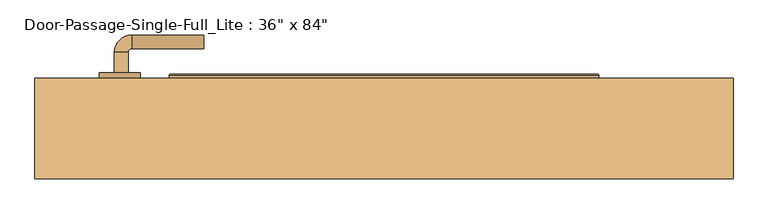
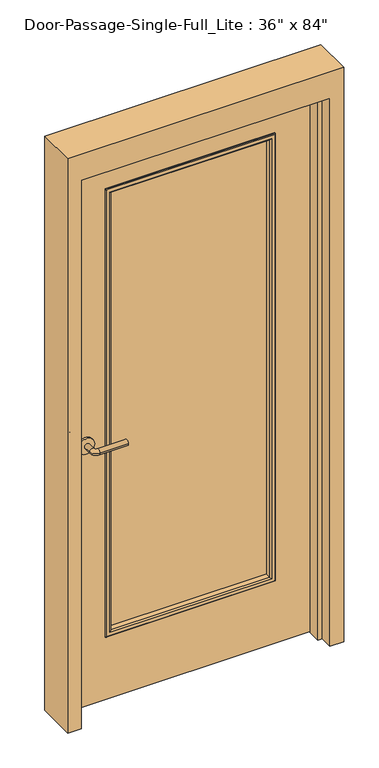
"""IFC4 building model written with IfcOpenShell, lengths in millimetres: door geometry."""

from ifc_helpers import new_model, si_unit, point, frame, frame_2d, origin, place, context, project, spatial, polyline, circle_curve, ellipse_curve, trimmed, segment, composite_curve, outline, extrude, faceted_brep, source, transform, mapped, element, save
from ifc_brep_helpers import plane_surface, cylinder_surface, revolved_surface, advanced_brep


def door_dac99271(model_context):
    return source(origin(), model_context, "Body", "SolidModel", [
        advanced_brep(
        [(-392.190625, 15.8125, 1016.0), (-372.190625, 15.8125, 1016.0), (-372.190625, -14.1875, 1016.0), (-392.190625, -14.1875, 1016.0), (-367.190625, -19.1875, 1016.0), (-367.190625, -39.1875, 1016.0), (-262.190625, -39.1875, 1016.0), (-262.190625, -19.1875, 1016.0)],
        [
            (0, 1, circle_curve(frame((-382.190625, 15.8125, 1016.0), z_axis=(0.0, 1.0, 0.0), x_axis=(1.0, 0.0, 0.0)), 10.0)),
            (1, 0, circle_curve(frame((-382.190625, 15.8125, 1016.0), z_axis=(0.0, 1.0, 0.0), x_axis=(1.0, 0.0, 0.0)), 10.0)),
            (1, 2),
            (2, 3, circle_curve(frame((-382.190625, -14.1875, 1016.0), z_axis=(0.0, 1.0, 0.0), x_axis=(1.0, 0.0, 0.0)), 10.0)),
            (3, 0),
            (3, 2, circle_curve(frame((-382.190625, -14.1875, 1016.0), z_axis=(0.0, 1.0, 0.0), x_axis=(1.0, 0.0, 0.0)), 10.0)),
            (4, 5, circle_curve(frame((-367.190625, -29.1875, 1016.0), z_axis=(-1.0, 0.0, 0.0), x_axis=(0.0, 1.0, 0.0)), 10.0)),
            (5, 3, circle_curve(frame((-367.190625, -14.1875, 1016.0), z_axis=(0.0, 0.0, -1.0), x_axis=(-1.0, 0.0, 0.0)), 25.0)),
            (2, 4, circle_curve(frame((-367.190625, -14.1875, 1016.0), z_axis=(0.0, 0.0, 1.0), x_axis=(-1.0, 0.0, 0.0)), 5.0)),
            (5, 4, circle_curve(frame((-367.190625, -29.1875, 1016.0), z_axis=(-1.0, 0.0, 0.0), x_axis=(0.0, 1.0, 0.0)), 10.0)),
            (6, 7, circle_curve(frame((-262.190625, -29.1875, 1016.0), z_axis=(1.0, 0.0, 0.0), x_axis=(0.0, 1.0, 0.0)), 10.0)),
            (7, 6, circle_curve(frame((-262.190625, -29.1875, 1016.0), z_axis=(1.0, 0.0, 0.0), x_axis=(0.0, 1.0, 0.0)), 10.0)),
            (4, 7),
            (6, 5),
        ],
        [
            plane_surface(frame((-382.190625, 15.8125, 1016.0), z_axis=(0.0, 1.0, 0.0), x_axis=(0.0, 0.0, 1.0))),
            cylinder_surface(frame((-382.190625, 15.8125, 1016.0), z_axis=(0.0, 1.0, 0.0), x_axis=(1.0, 0.0, 0.0)), 10.0),
            revolved_surface(trimmed(ellipse_curve(frame((-382.190625, -14.1875, 1016.0), z_axis=(0.0, -1.0, 0.0), x_axis=(1.0, 0.0, 0.0)), 10.0, 10.0), [point((-392.190625, -14.1875, 1016.0))], [point((-372.190625, -14.1875, 1016.0))], True, "CARTESIAN"), (-367.190625, -14.1875, 1016.0), (0.0, 0.0, -1.0)),
            revolved_surface(trimmed(ellipse_curve(frame((-382.190625, -14.1875, 1016.0), z_axis=(0.0, -1.0, 0.0), x_axis=(1.0, 0.0, 0.0)), 10.0, 10.0), [point((-372.190625, -14.1875, 1016.0))], [point((-392.190625, -14.1875, 1016.0))], True, "CARTESIAN"), (-367.190625, -14.1875, 1016.0), (0.0, 0.0, -1.0)),
            plane_surface(frame((-262.190625, -29.1875, 1016.0), z_axis=(1.0, 0.0, 0.0), x_axis=(0.0, 0.0, 1.0))),
            cylinder_surface(frame((-367.190625, -29.1875, 1016.0), z_axis=(-1.0, 0.0, 0.0), x_axis=(0.0, 1.0, 0.0)), 10.0),
        ],
        [
            (0, [[1, 2]]),
            (1, [[3, 4, 5, -2]]),
            (1, [[-5, 6, -3, -1]]),
            (2, [[7, 8, -4, 9]]),
            (3, [[10, -9, -6, -8]]),
            (4, [[11, 12]]),
            (5, [[13, -11, 14, -7]]),
            (5, [[-14, -12, -13, -10]]),
        ],
    ),
        extrude(outline(composite_curve([segment(trimmed(circle_curve(frame_2d((1016.0, -384.690625)), 30.0), [point((1016.0, -414.690625))], [point((1016.0, -354.690625))], False, "CARTESIAN"), True, "CONTINUOUS"), segment(trimmed(circle_curve(frame_2d((1016.0, -384.690625)), 30.0), [point((1016.0, -354.690625))], [point((1016.0, -414.690625))], False, "CARTESIAN"), True, "CONTINUOUS")], self_intersect=False)), frame((0.0, 15.8125, 0.0), z_axis=(0.0, 1.0, 0.0), x_axis=(0.0, 0.0, 1.0)), (0.0, 0.0, 1.0), 8.0),
        advanced_brep(
        [(-392.190625, 76.2625, 1016.0), (-372.190625, 76.2625, 1016.0), (-392.190625, 106.2625, 1016.0), (-372.190625, 106.2625, 1016.0), (-367.190625, 111.2625, 1016.0), (-367.190625, 131.2625, 1016.0), (-262.190625, 131.2625, 1016.0), (-262.190625, 111.2625, 1016.0)],
        [
            (0, 1, circle_curve(frame((-382.190625, 76.2625, 1016.0), z_axis=(0.0, -1.0, 0.0), x_axis=(1.0, 0.0, 0.0)), 10.0)),
            (1, 0, circle_curve(frame((-382.190625, 76.2625, 1016.0), z_axis=(0.0, -1.0, 0.0), x_axis=(1.0, 0.0, 0.0)), 10.0)),
            (0, 2),
            (2, 3, circle_curve(frame((-382.190625, 106.2625, 1016.0), z_axis=(0.0, -1.0, 0.0), x_axis=(1.0, 0.0, 0.0)), 10.0)),
            (3, 1),
            (3, 2, circle_curve(frame((-382.190625, 106.2625, 1016.0), z_axis=(0.0, -1.0, 0.0), x_axis=(1.0, 0.0, 0.0)), 10.0)),
            (4, 3, circle_curve(frame((-367.190625, 106.2625, 1016.0), z_axis=(0.0, 0.0, 1.0), x_axis=(-1.0, 0.0, 0.0)), 5.0)),
            (2, 5, circle_curve(frame((-367.190625, 106.2625, 1016.0), z_axis=(0.0, 0.0, -1.0), x_axis=(-1.0, 0.0, 0.0)), 25.0)),
            (5, 4, circle_curve(frame((-367.190625, 121.2625, 1016.0), z_axis=(-1.0, 0.0, 0.0), x_axis=(0.0, -1.0, 0.0)), 10.0)),
            (4, 5, circle_curve(frame((-367.190625, 121.2625, 1016.0), z_axis=(-1.0, 0.0, 0.0), x_axis=(0.0, -1.0, 0.0)), 10.0)),
            (6, 7, circle_curve(frame((-262.190625, 121.2625, 1016.0), z_axis=(1.0, 0.0, 0.0), x_axis=(0.0, -1.0, 0.0)), 10.0)),
            (7, 6, circle_curve(frame((-262.190625, 121.2625, 1016.0), z_axis=(1.0, 0.0, 0.0), x_axis=(0.0, -1.0, 0.0)), 10.0)),
            (5, 6),
            (7, 4),
        ],
        [
            plane_surface(frame((-382.190625, 76.2625, 1016.0), z_axis=(0.0, -1.0, 0.0), x_axis=(0.0, 0.0, 1.0))),
            cylinder_surface(frame((-382.190625, 76.2625, 1016.0), z_axis=(0.0, -1.0, 0.0), x_axis=(1.0, 0.0, 0.0)), 10.0),
            revolved_surface(trimmed(ellipse_curve(frame((-382.190625, 106.2625, 1016.0), z_axis=(0.0, -1.0, 0.0), x_axis=(1.0, 0.0, 0.0)), 10.0, 10.0), [point((-392.190625, 106.2625, 1016.0))], [point((-372.190625, 106.2625, 1016.0))], True, "CARTESIAN"), (-367.190625, 106.2625, 1016.0), (0.0, 0.0, -1.0)),
            revolved_surface(trimmed(ellipse_curve(frame((-382.190625, 106.2625, 1016.0), z_axis=(0.0, -1.0, 0.0), x_axis=(1.0, 0.0, 0.0)), 10.0, 10.0), [point((-372.190625, 106.2625, 1016.0))], [point((-392.190625, 106.2625, 1016.0))], True, "CARTESIAN"), (-367.190625, 106.2625, 1016.0), (0.0, 0.0, -1.0)),
            plane_surface(frame((-262.190625, 121.2625, 1016.0), z_axis=(1.0, 0.0, 0.0), x_axis=(0.0, 0.0, 1.0))),
            cylinder_surface(frame((-367.190625, 121.2625, 1016.0), z_axis=(-1.0, 0.0, 0.0), x_axis=(0.0, -1.0, 0.0)), 10.0),
        ],
        [
            (0, [[1, 2]]),
            (1, [[-1, 3, 4, 5]]),
            (1, [[-2, -5, 6, -3]]),
            (2, [[7, -4, 8, 9]]),
            (3, [[-8, -6, -7, 10]]),
            (4, [[11, 12]]),
            (5, [[-9, 13, -12, 14]]),
            (5, [[-10, -14, -11, -13]]),
        ],
    ),
        extrude(outline(composite_curve([segment(trimmed(circle_curve(frame_2d((1016.0, -384.690625)), 30.0), [point((1016.0, -414.690625))], [point((1016.0, -354.690625))], False, "CARTESIAN"), True, "CONTINUOUS"), segment(trimmed(circle_curve(frame_2d((1016.0, -384.690625)), 30.0), [point((1016.0, -354.690625))], [point((1016.0, -414.690625))], False, "CARTESIAN"), True, "CONTINUOUS")], self_intersect=False)), frame((0.0, 68.2625, 0.0), z_axis=(0.0, 1.0, 0.0), x_axis=(0.0, 0.0, 1.0)), (0.0, 0.0, 1.0), 8.0),
        extrude(outline(polyline([(304.8, 42.8625), (-304.8, 42.8625), (-304.8, 49.2125), (304.8, 49.2125), (304.8, 42.8625)])), frame((0.0, 0.0, 254.0), z_axis=(0.0, 0.0, 1.0), x_axis=(1.0, 0.0, 0.0)), (0.0, 0.0, 1.0), 1727.2),
        faceted_brep([(457.2, 19.05, 0.0), (457.2, 68.2625, 0.0), (508.0, 68.2625, 0.0), (508.0, -77.7875, 0.0), (457.2, -77.7875, 0.0), (457.2, -28.575, 0.0), (441.325, -28.575, 0.0), (441.325, 19.05, 0.0), (457.2, 19.05, 2133.6), (457.2, 68.2625, 2133.6), (-457.2, 68.2625, 2133.6), (-457.2, 68.2625, 0.0), (-508.0, 68.2625, 0.0), (-508.0, 68.2625, 2235.2), (508.0, 68.2625, 2235.2), (508.0, -77.7875, 2235.2), (-508.0, -77.7875, 2235.2), (-508.0, -77.7875, 0.0), (-457.2, -77.7875, 0.0), (-457.2, -77.7875, 2133.6), (457.2, -77.7875, 2133.6), (457.2, -28.575, 2133.6), (-457.2, -28.575, 2133.6), (-457.2, -28.575, 0.0), (-441.325, -28.575, 0.0), (-441.325, -28.575, 2117.725), (441.325, -28.575, 2117.725), (441.325, 19.05, 2117.725), (-441.325, 19.05, 2117.725), (-441.325, 19.05, 0.0), (-457.2, 19.05, 0.0), (-457.2, 19.05, 2133.6)], [[[0, 1, 2, 3, 4, 5, 6, 7]], [[1, 0, 8, 9]], [[2, 1, 9, 10, 11, 12, 13, 14]], [[3, 2, 14, 15]], [[4, 3, 15, 16, 17, 18, 19, 20]], [[5, 4, 20, 21]], [[6, 5, 21, 22, 23, 24, 25, 26]], [[7, 6, 26, 27]], [[0, 7, 27, 28, 29, 30, 31, 8]], [[9, 8, 31, 10]], [[20, 19, 22, 21]], [[26, 25, 28, 27]], [[12, 11, 30, 29, 24, 23, 18, 17]], [[11, 10, 31, 30]], [[13, 12, 17, 16]], [[19, 18, 23, 22]], [[25, 24, 29, 28]], [[15, 14, 13, 16]]]),
        extrude(outline(polyline([(2133.6, -457.2), (0.0, -457.2), (0.0, 457.2), (2133.6, 457.2), (2133.6, -457.2)]), holes=[polyline([(1981.2, -304.8), (1981.2, 304.8), (254.0, 304.8), (254.0, -304.8), (1981.2, -304.8)])]), frame((0.0, 23.8125, 0.0), z_axis=(0.0, 1.0, 0.0), x_axis=(0.0, 0.0, 1.0)), (0.0, 0.0, 1.0), 44.45),
        advanced_brep(
        [(-304.8, 49.2125, 1981.2), (-304.8, 68.2625, 1981.2), (-304.8, 68.2625, 254.0), (-304.8, 49.2125, 254.0), (-292.8, 69.2625, 1969.2), (-292.8, 49.2125, 1969.2), (-292.8, 49.2125, 266.0), (-292.8, 69.2625, 266.0), (-297.8, 74.2625, 1974.2), (-297.8, 74.2625, 261.0), (-312.8, 72.2625, 1989.2), (-310.8, 74.2625, 1987.2), (-310.8, 74.2625, 248.0), (-312.8, 72.2625, 246.0), (-312.8, 68.2625, 1989.2), (-312.8, 68.2625, 246.0), (304.8, 68.2625, 254.0), (304.8, 49.2125, 254.0), (292.8, 49.2125, 266.0), (292.8, 69.2625, 266.0), (297.8, 74.2625, 261.0), (310.8, 74.2625, 248.0), (312.8, 72.2625, 246.0), (312.8, 68.2625, 246.0), (304.8, 68.2625, 1981.2), (304.8, 49.2125, 1981.2), (292.8, 49.2125, 1969.2), (292.8, 69.2625, 1969.2), (297.8, 74.2625, 1974.2), (310.8, 74.2625, 1987.2), (312.8, 72.2625, 1989.2), (312.8, 68.2625, 1989.2)],
        [
            (0, 1),
            (1, 2),
            (2, 3),
            (3, 0),
            (4, 5),
            (5, 6),
            (6, 7),
            (7, 4),
            (8, 4, ellipse_curve(frame((-297.8, 69.2625, 1974.2), z_axis=(-0.7071067811865475, 0.0, -0.7071067811865475), x_axis=(-0.7071067811865474, 0.0, 0.7071067811865476)), 7.0710678, 5.0)),
            (7, 9, ellipse_curve(frame((-297.8, 69.2625, 261.0), z_axis=(-0.7071067811865475, 0.0, 0.7071067811865475), x_axis=(0.7071067811865474, 0.0, 0.7071067811865476)), 7.0710678, 5.0)),
            (9, 8),
            (10, 11, ellipse_curve(frame((-310.8, 72.2625, 1987.2), z_axis=(-0.7071067811865475, 0.0, -0.7071067811865475), x_axis=(-0.7071067811865474, 0.0, 0.7071067811865476)), 2.8284271, 2.0)),
            (11, 12),
            (12, 13, ellipse_curve(frame((-310.8, 72.2625, 248.0), z_axis=(-0.7071067811865475, 0.0, 0.7071067811865475), x_axis=(0.7071067811865474, 0.0, 0.7071067811865476)), 2.8284271, 2.0)),
            (13, 10),
            (14, 10),
            (13, 15),
            (15, 14),
            (2, 16),
            (16, 17),
            (17, 3),
            (6, 18),
            (18, 19),
            (19, 7),
            (19, 20, ellipse_curve(frame((297.8, 69.2625, 261.0), z_axis=(-0.7071067811865475, 0.0, -0.7071067811865475), x_axis=(-0.7071067811865476, 0.0, 0.7071067811865474)), 7.0710678, 5.0)),
            (20, 9),
            (12, 21),
            (21, 22, ellipse_curve(frame((310.8, 72.2625, 248.0), z_axis=(-0.7071067811865475, 0.0, -0.7071067811865475), x_axis=(-0.7071067811865476, 0.0, 0.7071067811865474)), 2.8284271, 2.0)),
            (22, 13),
            (22, 23),
            (23, 15),
            (16, 24),
            (24, 25),
            (25, 17),
            (18, 26),
            (26, 27),
            (27, 19),
            (27, 28, ellipse_curve(frame((297.8, 69.2625, 1974.2), z_axis=(0.7071067811865475, 0.0, -0.7071067811865475), x_axis=(-0.7071067811865474, 0.0, -0.7071067811865476)), 7.0710678, 5.0)),
            (28, 20),
            (21, 29),
            (29, 30, ellipse_curve(frame((310.8, 72.2625, 1987.2), z_axis=(0.7071067811865475, 0.0, -0.7071067811865475), x_axis=(-0.7071067811865474, 0.0, -0.7071067811865476)), 2.8284271, 2.0)),
            (30, 22),
            (30, 31),
            (31, 23),
            (31, 14),
            (1, 24),
            (0, 25),
            (5, 26),
            (4, 27),
            (8, 28),
            (11, 29),
            (10, 30),
        ],
        [
            plane_surface(frame((-304.8, 68.2625, 1981.2), z_axis=(-1.0, 0.0, 0.0), x_axis=(0.0, 0.0, -1.0))),
            plane_surface(frame((-292.8, 49.2125, 1969.2), z_axis=(1.0, 0.0, 0.0), x_axis=(0.0, 0.0, -1.0))),
            cylinder_surface(frame((-297.8, 69.2625, 1981.2), z_axis=(0.0, 0.0, 1.0), x_axis=(-1.0, 0.0, 0.0)), 5.0),
            cylinder_surface(frame((-310.8, 72.2625, 1981.2), z_axis=(0.0, 0.0, 1.0), x_axis=(-1.0, 0.0, 0.0)), 2.0),
            plane_surface(frame((-312.8, 72.2625, 1989.2), z_axis=(-1.0, 0.0, 0.0), x_axis=(0.0, 0.0, -1.0))),
            plane_surface(frame((-304.8, 68.2625, 254.0), z_axis=(0.0, 0.0, -1.0), x_axis=(1.0, 0.0, 0.0))),
            plane_surface(frame((-292.8, 49.2125, 266.0), z_axis=(0.0, 0.0, 1.0), x_axis=(1.0, 0.0, 0.0))),
            cylinder_surface(frame((-304.8, 69.2625, 261.0), z_axis=(-1.0, 0.0, 0.0), x_axis=(0.0, 0.0, -1.0)), 5.0),
            cylinder_surface(frame((-304.8, 72.2625, 248.0), z_axis=(-1.0, 0.0, 0.0), x_axis=(0.0, 0.0, -1.0)), 2.0),
            plane_surface(frame((-312.8, 72.2625, 246.0), z_axis=(0.0, 0.0, -1.0), x_axis=(1.0, 0.0, 0.0))),
            plane_surface(frame((304.8, 68.2625, 254.0), z_axis=(1.0, 0.0, 0.0), x_axis=(0.0, 0.0, 1.0))),
            plane_surface(frame((292.8, 49.2125, 266.0), z_axis=(-1.0, 0.0, 0.0), x_axis=(0.0, 0.0, 1.0))),
            cylinder_surface(frame((297.8, 69.2625, 254.0), z_axis=(0.0, 0.0, -1.0), x_axis=(1.0, 0.0, 0.0)), 5.0),
            cylinder_surface(frame((310.8, 72.2625, 254.0), z_axis=(0.0, 0.0, -1.0), x_axis=(1.0, 0.0, 0.0)), 2.0),
            plane_surface(frame((312.8, 72.2625, 246.0), z_axis=(1.0, 0.0, 0.0), x_axis=(0.0, 0.0, 1.0))),
            plane_surface(frame((312.8, 68.2625, 1989.2), z_axis=(0.0, -1.0, 0.0), x_axis=(-1.0, 0.0, 0.0))),
            plane_surface(frame((304.8, 68.2625, 1981.2), z_axis=(0.0, 0.0, 1.0), x_axis=(-1.0, 0.0, 0.0))),
            plane_surface(frame((304.8, 49.2125, 1981.2), z_axis=(0.0, -1.0, 0.0), x_axis=(-1.0, 0.0, 0.0))),
            plane_surface(frame((292.8, 49.2125, 1969.2), z_axis=(0.0, 0.0, -1.0), x_axis=(-1.0, 0.0, 0.0))),
            cylinder_surface(frame((304.8, 69.2625, 1974.2), z_axis=(1.0, 0.0, 0.0), x_axis=(0.0, 0.0, 1.0)), 5.0),
            plane_surface(frame((297.8, 74.2625, 1974.2), z_axis=(0.0, 1.0, 0.0), x_axis=(-1.0, 0.0, 0.0))),
            cylinder_surface(frame((304.8, 72.2625, 1987.2), z_axis=(1.0, 0.0, 0.0), x_axis=(0.0, 0.0, 1.0)), 2.0),
            plane_surface(frame((312.8, 72.2625, 1989.2), z_axis=(0.0, 0.0, 1.0), x_axis=(-1.0, 0.0, 0.0))),
        ],
        [
            (0, [[1, 2, 3, 4]]),
            (1, [[5, 6, 7, 8]]),
            (2, [[9, -8, 10, 11]]),
            (3, [[12, 13, 14, 15]]),
            (4, [[16, -15, 17, 18]]),
            (5, [[-3, 19, 20, 21]]),
            (6, [[-7, 22, 23, 24]]),
            (7, [[-10, -24, 25, 26]]),
            (8, [[-14, 27, 28, 29]]),
            (9, [[-17, -29, 30, 31]]),
            (10, [[-20, 32, 33, 34]]),
            (11, [[-23, 35, 36, 37]]),
            (12, [[-25, -37, 38, 39]]),
            (13, [[-28, 40, 41, 42]]),
            (14, [[-30, -42, 43, 44]]),
            (15, [[-31, -44, 45, -18], [46, -32, -19, -2]]),
            (16, [[-33, -46, -1, 47]]),
            (17, [[-21, -34, -47, -4], [48, -35, -22, -6]]),
            (18, [[-36, -48, -5, 49]]),
            (19, [[-38, -49, -9, 50]]),
            (20, [[51, -40, -27, -13], [-26, -39, -50, -11]]),
            (21, [[-41, -51, -12, 52]]),
            (22, [[-43, -52, -16, -45]]),
        ],
    ),
        advanced_brep(
        [(-304.8, 42.8625, 254.0), (-304.8, 23.8125, 254.0), (-304.8, 23.8125, 1981.2), (-304.8, 42.8625, 1981.2), (-292.8, 22.8125, 266.0), (-292.8, 42.8625, 266.0), (-292.8, 42.8625, 1969.2), (-292.8, 22.8125, 1969.2), (-297.8, 17.8125, 261.0), (-297.8, 17.8125, 1974.2), (-312.8, 19.8125, 246.0), (-310.8, 17.8125, 248.0), (-310.8, 17.8125, 1987.2), (-312.8, 19.8125, 1989.2), (-312.8, 23.8125, 246.0), (-312.8, 23.8125, 1989.2), (304.8, 23.8125, 1981.2), (304.8, 42.8625, 1981.2), (292.8, 42.8625, 1969.2), (292.8, 22.8125, 1969.2), (297.8, 17.8125, 1974.2), (310.8, 17.8125, 1987.2), (312.8, 19.8125, 1989.2), (312.8, 23.8125, 1989.2), (304.8, 23.8125, 254.0), (304.8, 42.8625, 254.0), (292.8, 42.8625, 266.0), (292.8, 22.8125, 266.0), (297.8, 17.8125, 261.0), (310.8, 17.8125, 248.0), (312.8, 19.8125, 246.0), (312.8, 23.8125, 246.0)],
        [
            (0, 1),
            (1, 2),
            (2, 3),
            (3, 0),
            (4, 5),
            (5, 6),
            (6, 7),
            (7, 4),
            (8, 4, ellipse_curve(frame((-297.8, 22.8125, 261.0), z_axis=(-0.7071067811865475, 0.0, 0.7071067811865475), x_axis=(-0.7071067811865474, 0.0, -0.7071067811865476)), 7.0710678, 5.0)),
            (7, 9, ellipse_curve(frame((-297.8, 22.8125, 1974.2), z_axis=(-0.7071067811865475, 0.0, -0.7071067811865475), x_axis=(0.7071067811865474, 0.0, -0.7071067811865476)), 7.0710678, 5.0)),
            (9, 8),
            (10, 11, ellipse_curve(frame((-310.8, 19.8125, 248.0), z_axis=(-0.7071067811865475, 0.0, 0.7071067811865475), x_axis=(-0.7071067811865474, 0.0, -0.7071067811865476)), 2.8284271, 2.0)),
            (11, 12),
            (12, 13, ellipse_curve(frame((-310.8, 19.8125, 1987.2), z_axis=(-0.7071067811865475, 0.0, -0.7071067811865475), x_axis=(0.7071067811865474, 0.0, -0.7071067811865476)), 2.8284271, 2.0)),
            (13, 10),
            (14, 10),
            (13, 15),
            (15, 14),
            (2, 16),
            (16, 17),
            (17, 3),
            (6, 18),
            (18, 19),
            (19, 7),
            (19, 20, ellipse_curve(frame((297.8, 22.8125, 1974.2), z_axis=(-0.7071067811865475, 0.0, 0.7071067811865475), x_axis=(-0.7071067811865476, 0.0, -0.7071067811865474)), 7.0710678, 5.0)),
            (20, 9),
            (12, 21),
            (21, 22, ellipse_curve(frame((310.8, 19.8125, 1987.2), z_axis=(-0.7071067811865475, 0.0, 0.7071067811865475), x_axis=(-0.7071067811865476, 0.0, -0.7071067811865474)), 2.8284271, 2.0)),
            (22, 13),
            (22, 23),
            (23, 15),
            (16, 24),
            (24, 25),
            (25, 17),
            (18, 26),
            (26, 27),
            (27, 19),
            (27, 28, ellipse_curve(frame((297.8, 22.8125, 261.0), z_axis=(0.7071067811865475, 0.0, 0.7071067811865475), x_axis=(-0.7071067811865474, 0.0, 0.7071067811865476)), 7.0710678, 5.0)),
            (28, 20),
            (21, 29),
            (29, 30, ellipse_curve(frame((310.8, 19.8125, 248.0), z_axis=(0.7071067811865475, 0.0, 0.7071067811865475), x_axis=(-0.7071067811865474, 0.0, 0.7071067811865476)), 2.8284271, 2.0)),
            (30, 22),
            (30, 31),
            (31, 23),
            (31, 14),
            (1, 24),
            (0, 25),
            (5, 26),
            (4, 27),
            (8, 28),
            (11, 29),
            (10, 30),
        ],
        [
            plane_surface(frame((-304.8, 23.8125, 254.0), z_axis=(-1.0, 0.0, 0.0), x_axis=(0.0, 0.0, 1.0))),
            plane_surface(frame((-292.8, 42.8625, 266.0), z_axis=(1.0, 0.0, 0.0), x_axis=(0.0, 0.0, 1.0))),
            cylinder_surface(frame((-297.8, 22.8125, 254.0), z_axis=(0.0, 0.0, -1.0), x_axis=(-1.0, 0.0, 0.0)), 5.0),
            cylinder_surface(frame((-310.8, 19.8125, 254.0), z_axis=(0.0, 0.0, -1.0), x_axis=(-1.0, 0.0, 0.0)), 2.0),
            plane_surface(frame((-312.8, 19.8125, 246.0), z_axis=(-1.0, 0.0, 0.0), x_axis=(0.0, 0.0, 1.0))),
            plane_surface(frame((-304.8, 23.8125, 1981.2), z_axis=(0.0, 0.0, 1.0), x_axis=(1.0, 0.0, 0.0))),
            plane_surface(frame((-292.8, 42.8625, 1969.2), z_axis=(0.0, 0.0, -1.0), x_axis=(1.0, 0.0, 0.0))),
            cylinder_surface(frame((-304.8, 22.8125, 1974.2), z_axis=(-1.0, 0.0, 0.0), x_axis=(0.0, 0.0, 1.0)), 5.0),
            cylinder_surface(frame((-304.8, 19.8125, 1987.2), z_axis=(-1.0, 0.0, 0.0), x_axis=(0.0, 0.0, 1.0)), 2.0),
            plane_surface(frame((-312.8, 19.8125, 1989.2), z_axis=(0.0, 0.0, 1.0), x_axis=(1.0, 0.0, 0.0))),
            plane_surface(frame((304.8, 23.8125, 1981.2), z_axis=(1.0, 0.0, 0.0), x_axis=(0.0, 0.0, -1.0))),
            plane_surface(frame((292.8, 42.8625, 1969.2), z_axis=(-1.0, 0.0, 0.0), x_axis=(0.0, 0.0, -1.0))),
            cylinder_surface(frame((297.8, 22.8125, 1981.2), z_axis=(0.0, 0.0, 1.0), x_axis=(1.0, 0.0, 0.0)), 5.0),
            cylinder_surface(frame((310.8, 19.8125, 1981.2), z_axis=(0.0, 0.0, 1.0), x_axis=(1.0, 0.0, 0.0)), 2.0),
            plane_surface(frame((312.8, 19.8125, 1989.2), z_axis=(1.0, 0.0, 0.0), x_axis=(0.0, 0.0, -1.0))),
            plane_surface(frame((312.8, 23.8125, 246.0), z_axis=(0.0, 1.0, 0.0), x_axis=(-1.0, 0.0, 0.0))),
            plane_surface(frame((304.8, 23.8125, 254.0), z_axis=(0.0, 0.0, -1.0), x_axis=(-1.0, 0.0, 0.0))),
            plane_surface(frame((304.8, 42.8625, 254.0), z_axis=(0.0, 1.0, 0.0), x_axis=(-1.0, 0.0, 0.0))),
            plane_surface(frame((292.8, 42.8625, 266.0), z_axis=(0.0, 0.0, 1.0), x_axis=(-1.0, 0.0, 0.0))),
            cylinder_surface(frame((304.8, 22.8125, 261.0), z_axis=(1.0, 0.0, 0.0), x_axis=(0.0, 0.0, -1.0)), 5.0),
            plane_surface(frame((297.8, 17.8125, 261.0), z_axis=(0.0, -1.0, 0.0), x_axis=(-1.0, 0.0, 0.0))),
            cylinder_surface(frame((304.8, 19.8125, 248.0), z_axis=(1.0, 0.0, 0.0), x_axis=(0.0, 0.0, -1.0)), 2.0),
            plane_surface(frame((312.8, 19.8125, 246.0), z_axis=(0.0, 0.0, -1.0), x_axis=(-1.0, 0.0, 0.0))),
        ],
        [
            (0, [[1, 2, 3, 4]]),
            (1, [[5, 6, 7, 8]]),
            (2, [[9, -8, 10, 11]]),
            (3, [[12, 13, 14, 15]]),
            (4, [[16, -15, 17, 18]]),
            (5, [[-3, 19, 20, 21]]),
            (6, [[-7, 22, 23, 24]]),
            (7, [[-10, -24, 25, 26]]),
            (8, [[-14, 27, 28, 29]]),
            (9, [[-17, -29, 30, 31]]),
            (10, [[-20, 32, 33, 34]]),
            (11, [[-23, 35, 36, 37]]),
            (12, [[-25, -37, 38, 39]]),
            (13, [[-28, 40, 41, 42]]),
            (14, [[-30, -42, 43, 44]]),
            (15, [[-31, -44, 45, -18], [46, -32, -19, -2]]),
            (16, [[-33, -46, -1, 47]]),
            (17, [[-21, -34, -47, -4], [48, -35, -22, -6]]),
            (18, [[-36, -48, -5, 49]]),
            (19, [[-38, -49, -9, 50]]),
            (20, [[51, -40, -27, -13], [-26, -39, -50, -11]]),
            (21, [[-41, -51, -12, 52]]),
            (22, [[-43, -52, -16, -45]]),
        ],
    ),
    ])


if __name__ == "__main__":
    model = new_model("IFC4")
    model_context = context("Model", 3, world=origin())
    ifc_project = project(units=[si_unit("LENGTHUNIT", "METRE", prefix="MILLI")], contexts=[model_context])
    site = spatial("IfcSite", under=ifc_project)
    building = spatial("IfcBuilding", under=site)
    placement = place(None, origin())
    door_shape = door_dac99271(model_context)
    element("IfcDoor", 1, ObjectType="Door-Passage-Single-Full_Lite : 36\" x 84\"", at=placement, inside=building, context=model_context, shape_type="MappedRepresentation", body=[
        mapped(door_shape, transform((0.0, 0.0, 0.0), x_axis=(1.0, 0.0, 0.0), y_axis=(0.0, 1.0, 0.0), z_axis=(0.0, 0.0, 1.0))),
    ])
    save(model, "model.ifc")

# Revit data of these elements
# Type "Door-Passage-Single-Full_Lite : 36\" x 84\""
#   Type Mark = "52"
#   Assembly Code = "B2030100"
#   Analytic Construction = "Wooden"
#   Thickness = 0' - 1 3/4"
#   Thermal Resistance (R) = 2.5876 (h·ft²·°F)/BTU
#   Swing Angle [instance default] = 90.00°
#   Strike Height = 3' - 4"
#   Rough Width [instance default] = 3' - 4"
#   Rough Height [instance default] = 7' - 4"
#   MF Opening Height [instance default] = 0' - 4"
#   MF Opening Width [instance default] = 0' - 4"
#   Inset Calculate [instance default] = 0' - 4"
#   Masonry Inset [instance default] = 0' - 1"
#   Height = 7' - 0"
#   Width = 3' - 0"
#   Heat Transfer Coefficient (U) = 0.3865 BTU/(h·ft²·°F)
#   Masonry Frame Depth = 0' - 5 3/4"
#   Masonry Frame [instance default] = yes
#   Function = 1
#   Dry Wall Frame [instance default] = no
#   Panel Material = Wood - Birch
#   Glazing = Glass
#   Glass Stop Material = Metal - Paint Finish - Grey
#   Frame Material = Metal - Paint Finish - Grey
#   Door Handle Material = Aluminum
#   Visual Light Transmittance = 0
#   Solar Heat Gain Coefficient = 0
#   Wall Closure = (empty or 0)
# Element 1 (IfcDoor, "Door-Passage-Single-Full_Lite : 36\" x 84\"")
#   Inset Calculate = 0' - 3"
#   Masonry Inset = 0' - 0"
#   Materials on its faces: "Metal - Paint Finish - Grey", "Aluminum", "Wood - Birch", "Glass"
# Materials
#   "Wood - Birch": class "Wood", colour RGB 166 116 52, transparency 0, Cost = 0
#   "Glass": class "Glass", colour RGB 0 128 192, transparency 0.75, Description = "Soda Lime Glass", Cost = 0
#   "Metal - Paint Finish - Grey": class "Paint", colour RGB 104 104 104, transparency 0, Cost = 0
#   "Aluminum": class "Metal", colour RGB 247 247 247, transparency 0, Description = "Aluminum 6061", Cost = 0
